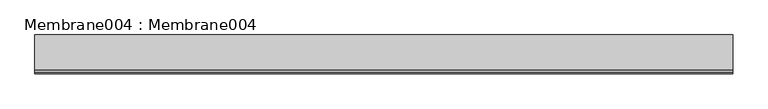
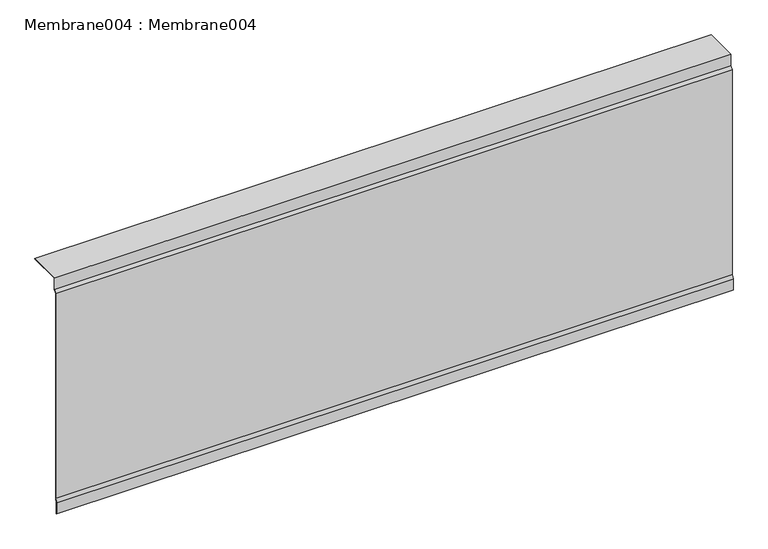
"""IFC4 building model written with IfcOpenShell, lengths in millimetres: proxy geometry, Membrane004 : Membrane004."""

from ifc_helpers import new_model, si_unit, frame, origin, place, context, project, spatial, polyline, outline, extrude, source, transform, mapped, element, save


def membrane004_membrane004_2a083e1b(model_context):
    return source(origin(), model_context, "Body", "SweptSolid", [
        extrude(outline(polyline([(-4311.4513818, 41057.992875), (-4311.4513818, 41056.992875), (-4409.9125977, 41056.992875), (-4409.9125977, 41022.2578125), (-4417.2509766, 41013.8828125), (-4417.2509766, 40372.6931249), (-4421.3365128, 40361.4678597), (-4421.3365128, 40326.5664062), (-4422.3365128, 40326.5664062), (-4422.3365128, 40361.6441867), (-4418.2509766, 40372.8694518), (-4418.2509766, 41014.258943), (-4410.9125977, 41022.6339431), (-4410.9125977, 41057.992875), (-4311.4513818, 41057.992875)])), frame((12383.0178845, 0.0, 0.0), z_axis=(1.0, 0.0, 0.0), x_axis=(0.0, 1.0, 0.0)), (0.0, 0.0, 1.0), 2000.0),
    ])


if __name__ == "__main__":
    model = new_model("IFC4")
    model_context = context("Model", 3, world=origin())
    ifc_project = project(units=[si_unit("LENGTHUNIT", "METRE", prefix="MILLI")], contexts=[model_context])
    site = spatial("IfcSite", under=ifc_project)
    building = spatial("IfcBuilding", under=site)
    placement = place(None, origin())
    membrane004_membrane004_shape = membrane004_membrane004_2a083e1b(model_context)
    element("IfcBuildingElementProxy", 1, Name="Membrane004 : Membrane004", ObjectType="Membrane004 : Membrane004", at=placement, inside=building, context=model_context, shape_type="MappedRepresentation", body=[
        mapped(membrane004_membrane004_shape, transform((0.0, 0.0, 0.0), x_axis=(1.0, 0.0, 0.0), y_axis=(0.0, 1.0, 0.0), z_axis=(0.0, 0.0, 1.0))),
    ])
    save(model, "model.ifc")

# Revit data of these elements
# Type "Membrane004 : Membrane004"
#   NameOverride = "Membrane004"
# Element 1 (IfcBuildingElementProxy, "Membrane004 : Membrane004")
#   Materials on its faces: "(2) LAYERS OF ICE & WATER SHIELD (BITUTHANE) UNDER STUCCO"
# Materials
#   "(2) LAYERS OF ICE & WATER SHIELD (BITUTHANE) UNDER STUCCO": class "Unassigned", colour RGB 186 255 159, transparency 0, Cost = 0
